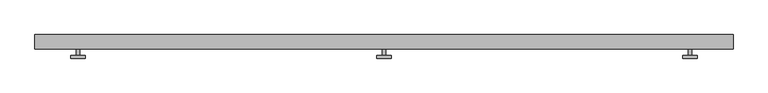
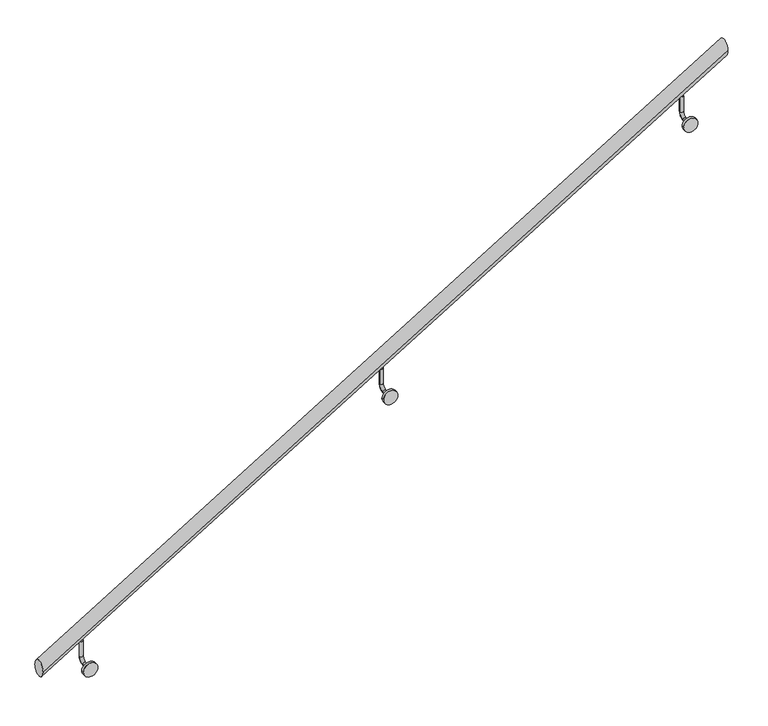
"""IFC4 building model written with IfcOpenShell, lengths in millimetres: railing geometry."""

from ifc_helpers import new_model, si_unit, point, frame, frame_2d, origin, place, context, project, spatial, circle_curve, ellipse_curve, trimmed, segment, composite_curve, outline, extrude, source, transform, mapped, element, save
from ifc_brep_helpers import plane_surface, cylinder_surface, revolved_surface, advanced_brep


def railing_5f4a1c35(model_context):
    return source(origin(), model_context, "Body", "SolidModel", [
        advanced_brep(
        [(-50191.7895023, 15484.3574868, 6395.7778144), (-50191.7895023, 15434.3574868, 6395.7778144), (-47761.7895023, 15484.3574868, 7876.1226419), (-47761.7895023, 15434.3574868, 7876.1226419)],
        [
            (0, 1, ellipse_curve(frame((-50191.7895023, 15459.3574868, 6395.7778144), z_axis=(-1.0, 0.0, 0.0), x_axis=(0.0, 0.0, -1.0)), 29.2736981, 25.0)),
            (1, 0, ellipse_curve(frame((-50191.7895023, 15459.3574868, 6395.7778144), z_axis=(-1.0, 0.0, 0.0), x_axis=(0.0, 0.0, -1.0)), 29.2736981, 25.0)),
            (2, 3, ellipse_curve(frame((-47761.7895023, 15459.3574868, 7876.1226419), z_axis=(1.0, 0.0, 0.0), x_axis=(0.0, 0.0, -1.0)), 29.2736981, 25.0)),
            (3, 2, ellipse_curve(frame((-47761.7895023, 15459.3574868, 7876.1226419), z_axis=(1.0, 0.0, 0.0), x_axis=(0.0, 0.0, -1.0)), 29.2736981, 25.0)),
            (0, 2),
            (3, 1),
        ],
        [
            plane_surface(frame((-50191.7895023, 15459.3574868, 6425.0515124), z_axis=(-1.0, 0.0, 0.0), x_axis=(0.0, 1.0, 0.0))),
            plane_surface(frame((-47761.7895023, 15459.3574868, 7905.39634), z_axis=(1.0, 0.0, 0.0), x_axis=(0.0, 1.0, 0.0))),
            cylinder_surface(frame((-50178.7830443, 15459.3574868, 6403.7012888), z_axis=(-0.8540089447440432, 0.0, -0.5202583226601627), x_axis=(0.0, -1.0, 0.0)), 25.0),
        ],
        [
            (0, [[1, 2]]),
            (1, [[3, 4]]),
            (2, [[-1, 5, -4, 6]]),
            (2, [[-2, -6, -3, -5]]),
        ],
    ),
        advanced_brep(
        [(-48983.1395023, 15459.3574868, 7096.1739262), (-48970.4395023, 15459.3574868, 7096.1739262), (-48983.1395023, 15459.3574868, 7039.0239262), (-48970.4395023, 15459.3574868, 7039.0239262), (-48970.4395023, 15440.3074868, 7019.9739262), (-48983.1395023, 15440.3074868, 7019.9739262), (-48983.1395023, 15411.7324868, 7019.9739262), (-48970.4395023, 15411.7324868, 7019.9739262)],
        [
            (0, 1, circle_curve(frame((-48976.7895023, 15459.3574868, 7096.1739262), z_axis=(0.0, 0.0, 1.0), x_axis=(1.0, 0.0, 0.0)), 6.35)),
            (1, 0, circle_curve(frame((-48976.7895023, 15459.3574868, 7096.1739262), z_axis=(0.0, 0.0, 1.0), x_axis=(1.0, 0.0, 0.0)), 6.35)),
            (0, 2),
            (2, 3, circle_curve(frame((-48976.7895023, 15459.3574868, 7039.0239262), z_axis=(0.0, 0.0, 1.0), x_axis=(1.0, 0.0, 0.0)), 6.35)),
            (3, 1),
            (3, 2, circle_curve(frame((-48976.7895023, 15459.3574868, 7039.0239262), z_axis=(0.0, 0.0, 1.0), x_axis=(1.0, 0.0, 0.0)), 6.35)),
            (4, 3, circle_curve(frame((-48970.4395023, 15440.3074868, 7039.0239262), z_axis=(1.0, 0.0, 0.0), x_axis=(0.0, 1.0, 0.0)), 19.05)),
            (2, 5, circle_curve(frame((-48983.1395023, 15440.3074868, 7039.0239262), z_axis=(-1.0, 0.0, 0.0), x_axis=(0.0, 1.0, 0.0)), 19.05)),
            (5, 4, circle_curve(frame((-48976.7895023, 15440.3074868, 7019.9739262), z_axis=(0.0, 1.0, 0.0), x_axis=(1.0, 0.0, 0.0)), 6.35)),
            (4, 5, circle_curve(frame((-48976.7895023, 15440.3074868, 7019.9739262), z_axis=(0.0, 1.0, 0.0), x_axis=(1.0, 0.0, 0.0)), 6.35)),
            (6, 7, circle_curve(frame((-48976.7895023, 15411.7324868, 7019.9739262), z_axis=(0.0, -1.0, 0.0), x_axis=(1.0, 0.0, 0.0)), 6.35)),
            (7, 6, circle_curve(frame((-48976.7895023, 15411.7324868, 7019.9739262), z_axis=(0.0, -1.0, 0.0), x_axis=(1.0, 0.0, 0.0)), 6.35)),
            (5, 6),
            (7, 4),
        ],
        [
            plane_surface(frame((-48970.4395023, 15459.3574868, 7096.1739262), z_axis=(0.0, 0.0, 1.0), x_axis=(0.0, -1.0, 0.0))),
            cylinder_surface(frame((-48976.7895023, 15459.3574868, 7096.1739262), z_axis=(0.0, 0.0, 1.0), x_axis=(1.0, 0.0, 0.0)), 6.35),
            revolved_surface(trimmed(ellipse_curve(frame((-48976.7895023, 15459.3574868, 7039.0239262), z_axis=(0.0, 0.0, 1.0), x_axis=(1.0, 0.0, 0.0)), 6.35, 6.35), [point((-48983.1395023, 15459.3574868, 7039.0239262))], [point((-48970.4395023, 15459.3574868, 7039.0239262))], True, "CARTESIAN"), (-48976.7895023, 15440.3074868, 7039.0239262), (-1.0, 0.0, 0.0)),
            revolved_surface(trimmed(ellipse_curve(frame((-48976.7895023, 15459.3574868, 7039.0239262), z_axis=(0.0, 0.0, 1.0), x_axis=(1.0, 0.0, 0.0)), 6.35, 6.35), [point((-48970.4395023, 15459.3574868, 7039.0239262))], [point((-48983.1395023, 15459.3574868, 7039.0239262))], True, "CARTESIAN"), (-48976.7895023, 15440.3074868, 7039.0239262), (-1.0, 0.0, 0.0)),
            plane_surface(frame((-48976.7895023, 15411.7324868, 7013.6239262), z_axis=(0.0, -1.0, 0.0), x_axis=(1.0, 0.0, 0.0))),
            cylinder_surface(frame((-48976.7895023, 15440.3074868, 7019.9739262), z_axis=(0.0, 1.0, 0.0), x_axis=(1.0, 0.0, 0.0)), 6.35),
        ],
        [
            (0, [[1, 2]]),
            (1, [[-1, 3, 4, 5]]),
            (1, [[-2, -5, 6, -3]]),
            (2, [[7, -4, 8, 9]]),
            (3, [[-8, -6, -7, 10]]),
            (4, [[11, 12]]),
            (5, [[-9, 13, -12, 14]]),
            (5, [[-10, -14, -11, -13]]),
        ],
    ),
        extrude(outline(composite_curve([segment(trimmed(circle_curve(frame_2d((7019.9739262, -48976.7895023)), 25.4), [point((7019.9739262, -48951.3895023))], [point((7019.9739262, -49002.1895023))], False, "CARTESIAN"), True, "CONTINUOUS"), segment(trimmed(circle_curve(frame_2d((7019.9739262, -48976.7895023)), 25.4), [point((7019.9739262, -49002.1895023))], [point((7019.9739262, -48951.3895023))], False, "CARTESIAN"), True, "CONTINUOUS")], self_intersect=False)), frame((0.0, 15402.2074868, 0.0), z_axis=(0.0, 1.0, 0.0), x_axis=(0.0, 0.0, 1.0)), (0.0, 0.0, 1.0), 9.525),
        advanced_brep(
        [(-47918.1395023, 15459.3574868, 7744.9670297), (-47905.4395023, 15459.3574868, 7744.9670297), (-47918.1395023, 15459.3574868, 7687.8170297), (-47905.4395023, 15459.3574868, 7687.8170297), (-47905.4395023, 15440.3074868, 7668.7670297), (-47918.1395023, 15440.3074868, 7668.7670297), (-47918.1395023, 15411.7324868, 7668.7670297), (-47905.4395023, 15411.7324868, 7668.7670297)],
        [
            (0, 1, circle_curve(frame((-47911.7895023, 15459.3574868, 7744.9670297), z_axis=(0.0, 0.0, 1.0), x_axis=(1.0, 0.0, 0.0)), 6.35)),
            (1, 0, circle_curve(frame((-47911.7895023, 15459.3574868, 7744.9670297), z_axis=(0.0, 0.0, 1.0), x_axis=(1.0, 0.0, 0.0)), 6.35)),
            (0, 2),
            (2, 3, circle_curve(frame((-47911.7895023, 15459.3574868, 7687.8170297), z_axis=(0.0, 0.0, 1.0), x_axis=(1.0, 0.0, 0.0)), 6.35)),
            (3, 1),
            (3, 2, circle_curve(frame((-47911.7895023, 15459.3574868, 7687.8170297), z_axis=(0.0, 0.0, 1.0), x_axis=(1.0, 0.0, 0.0)), 6.35)),
            (4, 3, circle_curve(frame((-47905.4395023, 15440.3074868, 7687.8170297), z_axis=(1.0, 0.0, 0.0), x_axis=(0.0, 1.0, 0.0)), 19.05)),
            (2, 5, circle_curve(frame((-47918.1395023, 15440.3074868, 7687.8170297), z_axis=(-1.0, 0.0, 0.0), x_axis=(0.0, 1.0, 0.0)), 19.05)),
            (5, 4, circle_curve(frame((-47911.7895023, 15440.3074868, 7668.7670297), z_axis=(0.0, 1.0, 0.0), x_axis=(1.0, 0.0, 0.0)), 6.35)),
            (4, 5, circle_curve(frame((-47911.7895023, 15440.3074868, 7668.7670297), z_axis=(0.0, 1.0, 0.0), x_axis=(1.0, 0.0, 0.0)), 6.35)),
            (6, 7, circle_curve(frame((-47911.7895023, 15411.7324868, 7668.7670297), z_axis=(0.0, -1.0, 0.0), x_axis=(1.0, 0.0, 0.0)), 6.35)),
            (7, 6, circle_curve(frame((-47911.7895023, 15411.7324868, 7668.7670297), z_axis=(0.0, -1.0, 0.0), x_axis=(1.0, 0.0, 0.0)), 6.35)),
            (5, 6),
            (7, 4),
        ],
        [
            plane_surface(frame((-47905.4395023, 15459.3574868, 7744.9670297), z_axis=(0.0, 0.0, 1.0), x_axis=(0.0, -1.0, 0.0))),
            cylinder_surface(frame((-47911.7895023, 15459.3574868, 7744.9670297), z_axis=(0.0, 0.0, 1.0), x_axis=(1.0, 0.0, 0.0)), 6.35),
            revolved_surface(trimmed(ellipse_curve(frame((-47911.7895023, 15459.3574868, 7687.8170297), z_axis=(0.0, 0.0, 1.0), x_axis=(1.0, 0.0, 0.0)), 6.35, 6.35), [point((-47918.1395023, 15459.3574868, 7687.8170297))], [point((-47905.4395023, 15459.3574868, 7687.8170297))], True, "CARTESIAN"), (-47911.7895023, 15440.3074868, 7687.8170297), (-1.0, 0.0, 0.0)),
            revolved_surface(trimmed(ellipse_curve(frame((-47911.7895023, 15459.3574868, 7687.8170297), z_axis=(0.0, 0.0, 1.0), x_axis=(1.0, 0.0, 0.0)), 6.35, 6.35), [point((-47905.4395023, 15459.3574868, 7687.8170297))], [point((-47918.1395023, 15459.3574868, 7687.8170297))], True, "CARTESIAN"), (-47911.7895023, 15440.3074868, 7687.8170297), (-1.0, 0.0, 0.0)),
            plane_surface(frame((-47911.7895023, 15411.7324868, 7662.4170297), z_axis=(0.0, -1.0, 0.0), x_axis=(1.0, 0.0, 0.0))),
            cylinder_surface(frame((-47911.7895023, 15440.3074868, 7668.7670297), z_axis=(0.0, 1.0, 0.0), x_axis=(1.0, 0.0, 0.0)), 6.35),
        ],
        [
            (0, [[1, 2]]),
            (1, [[-1, 3, 4, 5]]),
            (1, [[-2, -5, 6, -3]]),
            (2, [[7, -4, 8, 9]]),
            (3, [[-8, -6, -7, 10]]),
            (4, [[11, 12]]),
            (5, [[-9, 13, -12, 14]]),
            (5, [[-10, -14, -11, -13]]),
        ],
    ),
        extrude(outline(composite_curve([segment(trimmed(circle_curve(frame_2d((7668.7670297, -47911.7895023)), 25.4), [point((7668.7670297, -47886.3895023))], [point((7668.7670297, -47937.1895023))], False, "CARTESIAN"), True, "CONTINUOUS"), segment(trimmed(circle_curve(frame_2d((7668.7670297, -47911.7895023)), 25.4), [point((7668.7670297, -47937.1895023))], [point((7668.7670297, -47886.3895023))], False, "CARTESIAN"), True, "CONTINUOUS")], self_intersect=False)), frame((0.0, 15402.2074868, 0.0), z_axis=(0.0, 1.0, 0.0), x_axis=(0.0, 0.0, 1.0)), (0.0, 0.0, 1.0), 9.525),
        advanced_brep(
        [(-50048.1395023, 15459.3574868, 6447.3808228), (-50035.4395023, 15459.3574868, 6447.3808228), (-50048.1395023, 15459.3574868, 6390.2308228), (-50035.4395023, 15459.3574868, 6390.2308228), (-50035.4395023, 15440.3074868, 6371.1808228), (-50048.1395023, 15440.3074868, 6371.1808228), (-50048.1395023, 15411.7324868, 6371.1808228), (-50035.4395023, 15411.7324868, 6371.1808228)],
        [
            (0, 1, circle_curve(frame((-50041.7895023, 15459.3574868, 6447.3808228), z_axis=(0.0, 0.0, 1.0), x_axis=(1.0, 0.0, 0.0)), 6.35)),
            (1, 0, circle_curve(frame((-50041.7895023, 15459.3574868, 6447.3808228), z_axis=(0.0, 0.0, 1.0), x_axis=(1.0, 0.0, 0.0)), 6.35)),
            (0, 2),
            (2, 3, circle_curve(frame((-50041.7895023, 15459.3574868, 6390.2308228), z_axis=(0.0, 0.0, 1.0), x_axis=(1.0, 0.0, 0.0)), 6.35)),
            (3, 1),
            (3, 2, circle_curve(frame((-50041.7895023, 15459.3574868, 6390.2308228), z_axis=(0.0, 0.0, 1.0), x_axis=(1.0, 0.0, 0.0)), 6.35)),
            (4, 3, circle_curve(frame((-50035.4395023, 15440.3074868, 6390.2308228), z_axis=(1.0, 0.0, 0.0), x_axis=(0.0, 1.0, 0.0)), 19.05)),
            (2, 5, circle_curve(frame((-50048.1395023, 15440.3074868, 6390.2308228), z_axis=(-1.0, 0.0, 0.0), x_axis=(0.0, 1.0, 0.0)), 19.05)),
            (5, 4, circle_curve(frame((-50041.7895023, 15440.3074868, 6371.1808228), z_axis=(0.0, 1.0, 0.0), x_axis=(1.0, 0.0, 0.0)), 6.35)),
            (4, 5, circle_curve(frame((-50041.7895023, 15440.3074868, 6371.1808228), z_axis=(0.0, 1.0, 0.0), x_axis=(1.0, 0.0, 0.0)), 6.35)),
            (6, 7, circle_curve(frame((-50041.7895023, 15411.7324868, 6371.1808228), z_axis=(0.0, -1.0, 0.0), x_axis=(1.0, 0.0, 0.0)), 6.35)),
            (7, 6, circle_curve(frame((-50041.7895023, 15411.7324868, 6371.1808228), z_axis=(0.0, -1.0, 0.0), x_axis=(1.0, 0.0, 0.0)), 6.35)),
            (5, 6),
            (7, 4),
        ],
        [
            plane_surface(frame((-50035.4395023, 15459.3574868, 6447.3808228), z_axis=(0.0, 0.0, 1.0), x_axis=(0.0, -1.0, 0.0))),
            cylinder_surface(frame((-50041.7895023, 15459.3574868, 6447.3808228), z_axis=(0.0, 0.0, 1.0), x_axis=(1.0, 0.0, 0.0)), 6.35),
            revolved_surface(trimmed(ellipse_curve(frame((-50041.7895023, 15459.3574868, 6390.2308228), z_axis=(0.0, 0.0, 1.0), x_axis=(1.0, 0.0, 0.0)), 6.35, 6.35), [point((-50048.1395023, 15459.3574868, 6390.2308228))], [point((-50035.4395023, 15459.3574868, 6390.2308228))], True, "CARTESIAN"), (-50041.7895023, 15440.3074868, 6390.2308228), (-1.0, 0.0, 0.0)),
            revolved_surface(trimmed(ellipse_curve(frame((-50041.7895023, 15459.3574868, 6390.2308228), z_axis=(0.0, 0.0, 1.0), x_axis=(1.0, 0.0, 0.0)), 6.35, 6.35), [point((-50035.4395023, 15459.3574868, 6390.2308228))], [point((-50048.1395023, 15459.3574868, 6390.2308228))], True, "CARTESIAN"), (-50041.7895023, 15440.3074868, 6390.2308228), (-1.0, 0.0, 0.0)),
            plane_surface(frame((-50041.7895023, 15411.7324868, 6364.8308228), z_axis=(0.0, -1.0, 0.0), x_axis=(1.0, 0.0, 0.0))),
            cylinder_surface(frame((-50041.7895023, 15440.3074868, 6371.1808228), z_axis=(0.0, 1.0, 0.0), x_axis=(1.0, 0.0, 0.0)), 6.35),
        ],
        [
            (0, [[1, 2]]),
            (1, [[-1, 3, 4, 5]]),
            (1, [[-2, -5, 6, -3]]),
            (2, [[7, -4, 8, 9]]),
            (3, [[-8, -6, -7, 10]]),
            (4, [[11, 12]]),
            (5, [[-9, 13, -12, 14]]),
            (5, [[-10, -14, -11, -13]]),
        ],
    ),
        extrude(outline(composite_curve([segment(trimmed(circle_curve(frame_2d((6371.1808228, -50041.7895023)), 25.4), [point((6371.1808228, -50016.3895023))], [point((6371.1808228, -50067.1895023))], False, "CARTESIAN"), True, "CONTINUOUS"), segment(trimmed(circle_curve(frame_2d((6371.1808228, -50041.7895023)), 25.4), [point((6371.1808228, -50067.1895023))], [point((6371.1808228, -50016.3895023))], False, "CARTESIAN"), True, "CONTINUOUS")], self_intersect=False)), frame((0.0, 15402.2074868, 0.0), z_axis=(0.0, 1.0, 0.0), x_axis=(0.0, 0.0, 1.0)), (0.0, 0.0, 1.0), 9.525),
    ])


if __name__ == "__main__":
    model = new_model("IFC4")
    model_context = context("Model", 3, world=origin())
    ifc_project = project(units=[si_unit("LENGTHUNIT", "METRE", prefix="MILLI")], contexts=[model_context])
    site = spatial("IfcSite", under=ifc_project)
    building = spatial("IfcBuilding", under=site)
    placement = place(None, origin())
    railing_shape = railing_5f4a1c35(model_context)
    element("IfcRailing", 1, at=placement, inside=building, context=model_context, shape_type="MappedRepresentation", body=[
        mapped(railing_shape, transform((0.0, 0.0, 0.0), x_axis=(1.0, 0.0, 0.0), y_axis=(0.0, 1.0, 0.0), z_axis=(0.0, 0.0, 1.0))),
    ])
    save(model, "model.ifc")
